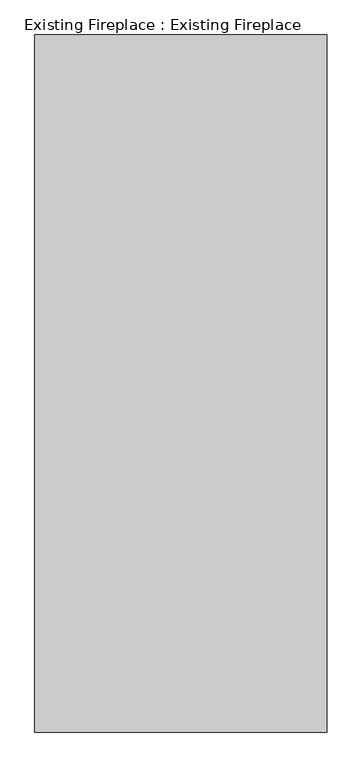
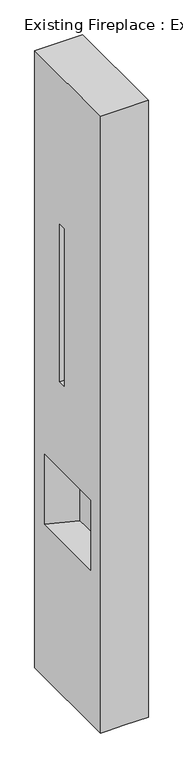
"""IFC4 building model written with IfcOpenShell, lengths in millimetres: proxy geometry, Existing Fireplace : Existing Fireplace."""

import ifcopenshell
import ifcopenshell.guid

model = None  # the IFC model being written
_history = None  # IfcOwnerHistory: only IFC2X3 demands one
_inside = {}  # id of a spatial element -> (the spatial element, [elements in it])
_under = {}  # id of a project, library or spatial element -> (it, [spatial elements below it])
_declared = {}  # id of a project -> (the project, [libraries it declares])
_typed = {}  # id of a type object -> (the type object, [elements of that type])
_made_of = {}  # id of a material, layer set ... -> (it, [elements and type objects made of it])


def new_model(schema):
    """Start an empty IFC model of exactly this schema.

    Asked for "IFC4X3", IfcOpenShell would pick the latest addendum, in which some entities
    have other attributes; the version numbers below select the first issue.
    IFC2X3 requires an IfcOwnerHistory on every rooted entity: one is made here for all.
    """
    global model, _history
    if schema == "IFC4X3":
        model = ifcopenshell.file(schema_version=(4, 3, 0, 0))
    else:
        model = ifcopenshell.file(schema=schema)
    _inside.clear()
    _under.clear()
    _declared.clear()
    _typed.clear()
    _made_of.clear()
    _history = None
    if model.schema == "IFC2X3":
        org = make("IfcOrganization", Name="unknown")
        user = make(
            "IfcPersonAndOrganization",
            ThePerson=make("IfcPerson", FamilyName="unknown"),
            TheOrganization=org,
        )
        app = make(
            "IfcApplication",
            ApplicationDeveloper=org,
            Version="unknown",
            ApplicationFullName="unknown",
            ApplicationIdentifier="unknown",
        )
        _history = make(
            "IfcOwnerHistory",
            OwningUser=user,
            OwningApplication=app,
            ChangeAction="ADDED",
            CreationDate=0,
        )
    return model


def make(cls, **values):
    """One entity of the class cls with the attributes given. An attribute that is None is left unset."""
    return model.create_entity(
        cls, **{name: value for name, value in values.items() if value is not None}
    )


def rooted(cls, **values):
    """An entity with a GlobalId (a new one), such as an element, a storey or a relation."""
    return make(cls, GlobalId=ifcopenshell.guid.new(), OwnerHistory=_history, **values)


def si_unit(unit_type, name, prefix=None):
    """IfcSIUnit, for example si_unit("LENGTHUNIT", "METRE", prefix="MILLI")."""
    return make("IfcSIUnit", UnitType=unit_type, Prefix=prefix, Name=name)


def assignment(units):
    """IfcUnitAssignment: the units of a project."""
    return None if units is None else make("IfcUnitAssignment", Units=units)


def point(xyz):
    """IfcCartesianPoint."""
    return None if xyz is None else make("IfcCartesianPoint", Coordinates=xyz)


def direction(xyz):
    """IfcDirection."""
    return None if xyz is None else make("IfcDirection", DirectionRatios=xyz)


def frame(location, z_axis=None, x_axis=None):
    """IfcAxis2Placement3D, a coordinate frame: its origin and axes. An axis left out is left unset."""
    return make(
        "IfcAxis2Placement3D",
        Location=point(location),
        Axis=direction(z_axis),
        RefDirection=direction(x_axis),
    )


def origin():
    """The frame at (0, 0, 0) with its axes left unset."""
    return frame((0.0, 0.0, 0.0))


def place(relative_to, where):
    """IfcLocalPlacement: puts the frame where relative to a parent placement (None: the world)."""
    return make(
        "IfcLocalPlacement", PlacementRelTo=relative_to, RelativePlacement=where
    )


def context(
    kind, dimensions, precision=None, world=None, true_north=None, identifier=None
):
    """IfcGeometricRepresentationContext, for example the 3D "Model" context."""
    return make(
        "IfcGeometricRepresentationContext",
        ContextIdentifier=identifier,
        ContextType=kind,
        CoordinateSpaceDimension=dimensions,
        Precision=precision,
        WorldCoordinateSystem=world,
        TrueNorth=true_north,
    )


def project(units=None, contexts=None):
    """IfcProject with its units and contexts."""
    return rooted(
        "IfcProject",
        Name="project",
        RepresentationContexts=contexts,
        UnitsInContext=assignment(units),
    )


def spatial(cls, under=None, at=None, **own):
    """A site, building, storey or space (cls), placed at a placement, below another one or the project."""
    s = rooted(cls, ObjectPlacement=at, **own)
    if under is not None:
        _under.setdefault(under.id(), (under, []))[1].append(s)
    return s


def faces_of(points, faces, orient=None, outer=None):
    """IfcFace entities. A face is a list of loops; a loop is a list of indices into points, from 0.

    orient and outer hold one flag for each loop. By default every Orientation is true, the
    first loop of a face is its IfcFaceOuterBound and the others are IfcFaceBound.
    """
    made = []
    for i, loops in enumerate(faces):
        bounds = []
        for j, loop in enumerate(loops):
            is_outer = j == 0 if outer is None else outer[i][j]
            bounds.append(
                make(
                    "IfcFaceOuterBound" if is_outer else "IfcFaceBound",
                    Bound=make("IfcPolyLoop", Polygon=[points[k] for k in loop]),
                    Orientation=True if orient is None else orient[i][j],
                )
            )
        made.append(make("IfcFace", Bounds=bounds))
    return made


def faceted_brep(points, faces, orient=None, outer=None, voids=None):
    """IfcFacetedBrep: a solid bounded by flat faces; with voids (closed shells), ...WithVoids."""
    shared = [point(p) for p in points]
    hull = make("IfcClosedShell", CfsFaces=faces_of(shared, faces, orient, outer))
    if voids is None:
        return make("IfcFacetedBrep", Outer=hull)
    return make(
        "IfcFacetedBrepWithVoids",
        Outer=hull,
        Voids=[
            make(cls, CfsFaces=faces_of(shared, fs, o, b)) for cls, fs, o, b in voids
        ],
    )


def shape(context_of_items, identifier, shape_type, items):
    """IfcShapeRepresentation: the items that make up one representation, for example the "Body"."""
    return make(
        "IfcShapeRepresentation",
        ContextOfItems=context_of_items,
        RepresentationIdentifier=identifier,
        RepresentationType=shape_type,
        Items=items,
    )


def source(mapping_origin, context_of_items, identifier, shape_type, items):
    """IfcRepresentationMap: a shape defined once, which mapped items show again and again."""
    return make(
        "IfcRepresentationMap",
        MappingOrigin=mapping_origin,
        MappedRepresentation=shape(context_of_items, identifier, shape_type, items),
    )


def transform(
    local_origin,
    x_axis=None,
    y_axis=None,
    z_axis=None,
    scale=None,
    scale2=None,
    scale3=None,
    uniform=True,
):
    """IfcCartesianTransformationOperator3D, or its non-uniform kind. x_axis, y_axis, z_axis: its Axis1, 2, 3."""
    if uniform:
        return make(
            "IfcCartesianTransformationOperator3D",
            Axis1=direction(x_axis),
            Axis2=direction(y_axis),
            LocalOrigin=point(local_origin),
            Scale=scale,
            Axis3=direction(z_axis),
        )
    return make(
        "IfcCartesianTransformationOperator3DnonUniform",
        Axis1=direction(x_axis),
        Axis2=direction(y_axis),
        LocalOrigin=point(local_origin),
        Scale=scale,
        Axis3=direction(z_axis),
        Scale2=scale2,
        Scale3=scale3,
    )


def mapped(mapping_source, mapping_target):
    """IfcMappedItem: shows the shape of a source again, moved by a transform."""
    return make(
        "IfcMappedItem", MappingSource=mapping_source, MappingTarget=mapping_target
    )


def made_of(thing, what):
    """Note that an element or type object is made of a material, layer set ...; save() writes the relation."""
    if what is not None:
        _made_of.setdefault(what.id(), (what, []))[1].append(thing)
    return thing


def element(
    cls,
    number,
    at=None,
    inside=None,
    cuts=None,
    type_object=None,
    material=None,
    context=None,
    identifier="Body",
    shape_type=None,
    held_by="IfcProductDefinitionShape",
    body=None,
    shapes=None,
    **own,
):
    """One element of the class cls, such as IfcWall. Its Tag is "e" and its number.

    at: its placement. inside: the storey or other place that contains it. cuts: it is an
    opening in that element (IfcRelVoidsElement). A single representation is given by context,
    identifier, shape_type and body (its items); several are given by shapes. held_by: the class
    of the entity that holds the representations. save() writes the other relations.
    """
    e = rooted(cls, Tag="e%d" % number, ObjectPlacement=at, **own)
    if body is not None:
        shapes = [shape(context, identifier, shape_type, body)]
    if shapes is not None:
        e.Representation = make(held_by, Representations=shapes)
    if inside is not None:
        _inside.setdefault(inside.id(), (inside, []))[1].append(e)
    if cuts is not None:
        rooted(
            "IfcRelVoidsElement", RelatingBuildingElement=cuts, RelatedOpeningElement=e
        )
    if type_object is not None:
        _typed.setdefault(type_object.id(), (type_object, []))[1].append(e)
    return made_of(e, material)


def aggregate(whole, parts):
    """IfcRelAggregates: a whole, such as a stair, and the parts it consists of."""
    return rooted("IfcRelAggregates", RelatingObject=whole, RelatedObjects=parts)


def save(model, path):
    """Write the relations noted so far, then the file.

    IfcRelAggregates (storeys below a building ...), IfcRelContainedInSpatialStructure (elements
    in a storey), IfcRelDefinesByType, IfcRelAssociatesMaterial and IfcRelDeclares: one each for
    every whole, place, type object, material and project.
    """
    for whole, parts in _under.values():
        aggregate(whole, parts)
    for where, things in _inside.values():
        rooted(
            "IfcRelContainedInSpatialStructure",
            RelatedElements=things,
            RelatingStructure=where,
        )
    for kind, things in _typed.values():
        rooted("IfcRelDefinesByType", RelatedObjects=things, RelatingType=kind)
    for what, things in _made_of.values():
        rooted("IfcRelAssociatesMaterial", RelatedObjects=things, RelatingMaterial=what)
    for by, libraries in _declared.values():
        rooted("IfcRelDeclares", RelatingContext=by, RelatedDefinitions=libraries)
    model.write(path)


def existing_fireplace_existing_fireplace_287aed51(model_context):
    return source(origin(), model_context, "Body", "Brep", [
        faceted_brep([(4450.2196932, 434.2888758, 8077.2), (3662.8196932, 434.2888758, 8077.2), (3662.8196932, -1445.3111242, 8077.2), (4450.2196932, -1445.3111242, 8077.2), (4450.2196932, 434.2888758, -2667.0), (4450.2196932, -1445.3111242, -2667.0), (4069.2196932, -1445.3111242, -2667.0), (3764.4196932, -1445.3111242, -2667.0), (3662.8196932, -1445.3111242, -2667.0), (3662.8196932, 434.2888758, -2667.0), (3764.4196932, 434.2888758, -2667.0), (4069.2196932, 434.2888758, -2667.0), (3662.8196932, 154.8888758, 0.0), (3662.8196932, 154.8888758, 1219.2), (3662.8196932, -1165.9111242, 1219.2), (3662.8196932, -1165.9111242, 0.0), (3662.8196932, -403.9111242, 5486.4), (3662.8196932, -403.9111242, 2743.2), (3662.8196932, -276.9111242, 2743.2), (3662.8196932, -276.9111242, 5486.4), (4145.4196932, -20.7631592, 1219.2), (4145.4196932, -990.2590891, 1219.2), (4145.4196932, -990.2590891, 0.0), (4145.4196932, -20.7631592, 0.0), (3767.2567114, -403.9111242, 5486.4), (3767.2567114, -403.9111242, 2743.2), (3767.2567114, -276.9111242, 2743.2), (3767.2567114, -276.9111242, 5486.4)], [[[0, 1, 2, 3]], [[4, 5, 6, 7, 8, 9, 10, 11]], [[1, 0, 4, 11, 10, 9]], [[2, 1, 9, 8], [12, 13, 14, 15], [16, 17, 18, 19]], [[3, 2, 8, 7, 6, 5]], [[0, 3, 5, 4]], [[14, 13, 20, 21]], [[15, 14, 21, 22]], [[21, 20, 23, 22]], [[13, 12, 23, 20]], [[12, 15, 22, 23]], [[24, 25, 17, 16]], [[26, 27, 19, 18]], [[25, 26, 18, 17]], [[25, 24, 27, 26]], [[27, 24, 16, 19]]]),
    ])


if __name__ == "__main__":
    model = new_model("IFC4")
    model_context = context("Model", 3, world=origin())
    ifc_project = project(units=[si_unit("LENGTHUNIT", "METRE", prefix="MILLI")], contexts=[model_context])
    site = spatial("IfcSite", under=ifc_project)
    building = spatial("IfcBuilding", under=site)
    placement = place(None, origin())
    existing_fireplace_existing_fireplace_shape = existing_fireplace_existing_fireplace_287aed51(model_context)
    element("IfcBuildingElementProxy", 1, Name="Existing Fireplace : Existing Fireplace", ObjectType="Existing Fireplace : Existing Fireplace", at=placement, inside=building, context=model_context, shape_type="MappedRepresentation", body=[
        mapped(existing_fireplace_existing_fireplace_shape, transform((0.0, 0.0, 0.0), x_axis=(1.0, 0.0, 0.0), y_axis=(0.0, 1.0, 0.0), z_axis=(0.0, 0.0, 1.0))),
    ])
    save(model, "model.ifc")
